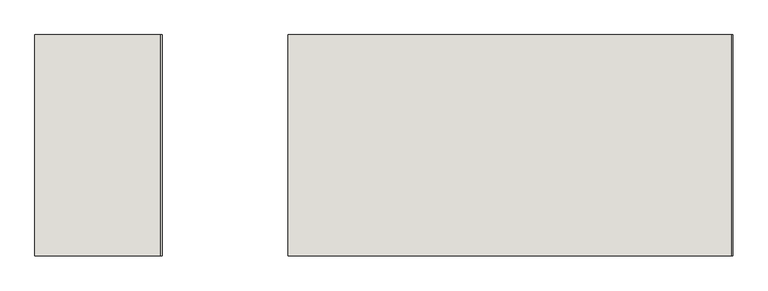
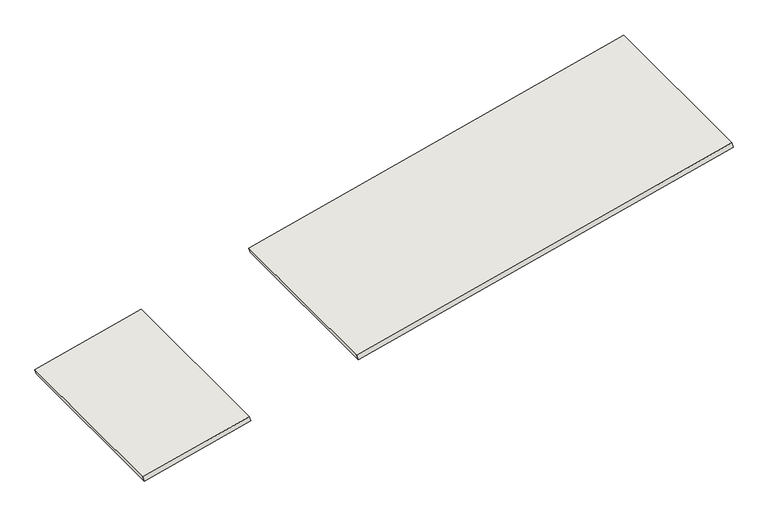
"""IFC4 building model written with IfcOpenShell, lengths in millimetres: wall geometry, BEADBOARD (EXT. EXPOSER RATING AT SOFFIT) : BEADBOARD (EXT. EXPOSER RATING AT SOFFIT)."""

from ifc_helpers import new_model, si_unit, frame, origin, place, context, project, spatial, polyline, outline, extrude, source, transform, mapped, element, save


def wall_9729bd50(model_context):
    return source(origin(), model_context, "Body", "SweptSolid", [
        extrude(outline(polyline([(0.0, -401.9898846), (0.0, 0.0), (685.8, 0.0), (685.8, -401.9898846), (0.0, -401.9898846)])), frame((17433.1004466, -2319.6634634, 2223.8920698), z_axis=(-0.24253562503632728, 0.0, 0.9701425001453333), x_axis=(0.0, 1.0, 0.0)), (0.0, 0.0, 1.0), 19.05),
        extrude(outline(polyline([(0.0, -1416.158302), (0.0, 0.0), (685.8, 0.0), (685.8, -1416.158302), (0.0, -1416.158302)])), frame((18217.2073089, -2319.6634634, 2419.9187854), z_axis=(-0.24253562503632706, 0.0, 0.9701425001453334), x_axis=(0.0, 1.0, 0.0)), (0.0, 0.0, 1.0), 19.05),
    ])


if __name__ == "__main__":
    model = new_model("IFC4")
    model_context = context("Model", 3, world=origin())
    ifc_project = project(units=[si_unit("LENGTHUNIT", "METRE", prefix="MILLI")], contexts=[model_context])
    site = spatial("IfcSite", under=ifc_project)
    building = spatial("IfcBuilding", under=site)
    placement = place(None, origin())
    wall_shape = wall_9729bd50(model_context)
    element("IfcWall", 1, ObjectType="BEADBOARD (EXT. EXPOSER RATING AT SOFFIT) : BEADBOARD (EXT. EXPOSER RATING AT SOFFIT)", at=placement, inside=building, context=model_context, shape_type="MappedRepresentation", body=[
        mapped(wall_shape, transform((0.0, 0.0, 0.0), x_axis=(1.0, 0.0, 0.0), y_axis=(0.0, 1.0, 0.0), z_axis=(0.0, 0.0, 1.0))),
    ])
    save(model, "model.ifc")

# Revit data of these elements
# Element 1 (IfcWall, "BEADBOARD (EXT. EXPOSER RATING AT SOFFIT) : BEADBOARD (EXT. EXPOSER RATING AT SOFFIT)")
#   Materials on its faces: "PLYTANIUM PLYWOOD EXTERIOR SIDING T1-11 - 4\" O.C. - STAIN T.B.D."
# Materials
#   "PLYTANIUM PLYWOOD EXTERIOR SIDING T1-11 - 4\" O.C. - STAIN T.B.D.": class "Unassigned", colour RGB 196 177 123, transparency 0, Cost = 0
